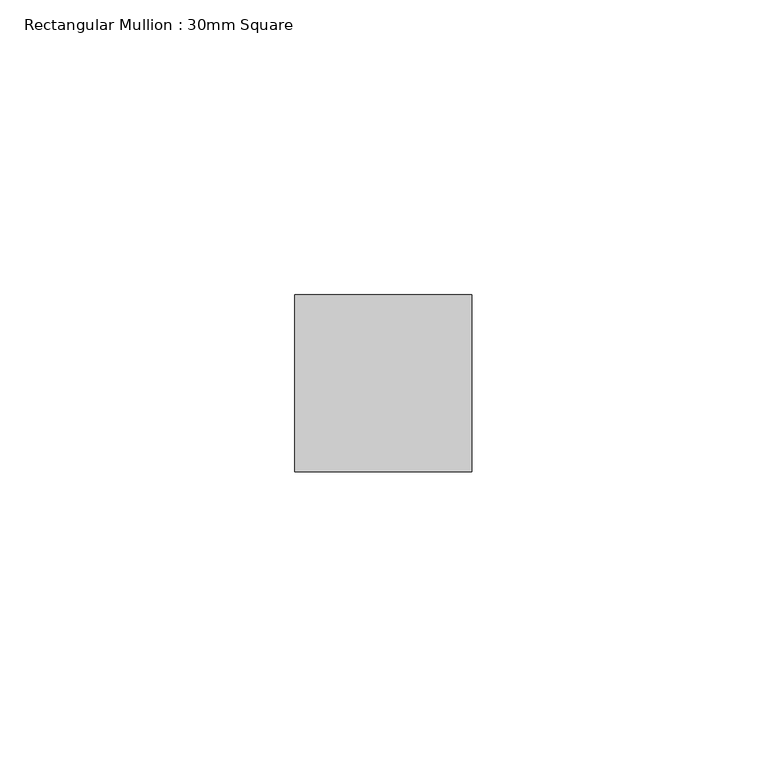
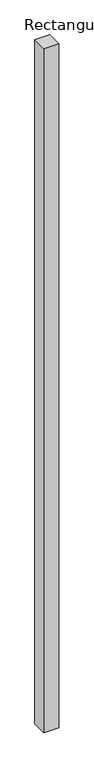
"""IFC4 building model written with IfcOpenShell, lengths in millimetres: member geometry, Rectangular Mullion : 30mm Square."""

from ifc_helpers import new_model, si_unit, frame, origin, place, context, project, spatial, polyline, outline, extrude, source, transform, mapped, element, save


def rectangular_mullion_30mm_square_68e71f7f(model_context):
    return source(origin(), model_context, "Body", "SweptSolid", [
        extrude(outline(polyline([(15.0, 15.0), (15.0, -15.0), (-15.0, -15.0), (-15.0, 15.0), (15.0, 15.0)])), frame((0.0, 0.0, -1442.9441358), z_axis=(0.0, 0.0, 1.0), x_axis=(1.0, 0.0, 0.0)), (0.0, 0.0, 1.0), 1442.9441358),
    ])


if __name__ == "__main__":
    model = new_model("IFC4")
    model_context = context("Model", 3, world=origin())
    ifc_project = project(units=[si_unit("LENGTHUNIT", "METRE", prefix="MILLI")], contexts=[model_context])
    site = spatial("IfcSite", under=ifc_project)
    building = spatial("IfcBuilding", under=site)
    placement = place(None, origin())
    rectangular_mullion_30mm_square_shape = rectangular_mullion_30mm_square_68e71f7f(model_context)
    element("IfcMember", 1, ObjectType="Rectangular Mullion : 30mm Square", at=placement, inside=building, context=model_context, shape_type="MappedRepresentation", body=[
        mapped(rectangular_mullion_30mm_square_shape, transform((0.0, 0.0, 0.0), x_axis=(1.0, 0.0, 0.0), y_axis=(0.0, 1.0, 0.0), z_axis=(0.0, 0.0, 1.0))),
    ])
    save(model, "model.ifc")

# Revit data of these elements
# Type "Rectangular Mullion : 30mm Square"
#   built-in parameter 1007304 = 0.0984252 (stored number, unit not read)
#   built-in parameter 1007301 = 0.0492126 (stored number, unit not read)
#   built-in parameter 1007300 = 0.0492126 (stored number, unit not read)
# Element 1 (IfcMember, "Rectangular Mullion : 30mm Square")
#   Materials on its faces: "Aluminum"
# Materials
#   "Aluminum": class "Metal", colour RGB 244 244 244, transparency 0, Description = "Aluminum 6061", Cost = 0
